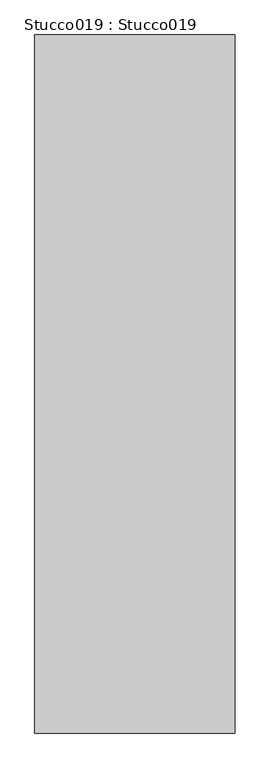
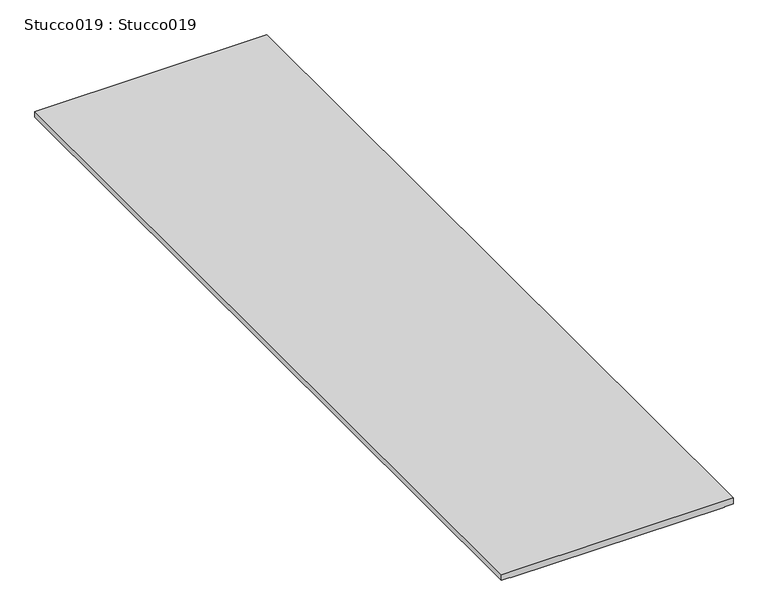
"""IFC4 building model written with IfcOpenShell, lengths in millimetres: proxy geometry, Stucco019 : Stucco019."""

import ifcopenshell
import ifcopenshell.guid

model = None  # the IFC model being written
_history = None  # IfcOwnerHistory: only IFC2X3 demands one
_inside = {}  # id of a spatial element -> (the spatial element, [elements in it])
_under = {}  # id of a project, library or spatial element -> (it, [spatial elements below it])
_declared = {}  # id of a project -> (the project, [libraries it declares])
_typed = {}  # id of a type object -> (the type object, [elements of that type])
_made_of = {}  # id of a material, layer set ... -> (it, [elements and type objects made of it])


def new_model(schema):
    """Start an empty IFC model of exactly this schema.

    Asked for "IFC4X3", IfcOpenShell would pick the latest addendum, in which some entities
    have other attributes; the version numbers below select the first issue.
    IFC2X3 requires an IfcOwnerHistory on every rooted entity: one is made here for all.
    """
    global model, _history
    if schema == "IFC4X3":
        model = ifcopenshell.file(schema_version=(4, 3, 0, 0))
    else:
        model = ifcopenshell.file(schema=schema)
    _inside.clear()
    _under.clear()
    _declared.clear()
    _typed.clear()
    _made_of.clear()
    _history = None
    if model.schema == "IFC2X3":
        org = make("IfcOrganization", Name="unknown")
        user = make(
            "IfcPersonAndOrganization",
            ThePerson=make("IfcPerson", FamilyName="unknown"),
            TheOrganization=org,
        )
        app = make(
            "IfcApplication",
            ApplicationDeveloper=org,
            Version="unknown",
            ApplicationFullName="unknown",
            ApplicationIdentifier="unknown",
        )
        _history = make(
            "IfcOwnerHistory",
            OwningUser=user,
            OwningApplication=app,
            ChangeAction="ADDED",
            CreationDate=0,
        )
    return model


def make(cls, **values):
    """One entity of the class cls with the attributes given. An attribute that is None is left unset."""
    return model.create_entity(
        cls, **{name: value for name, value in values.items() if value is not None}
    )


def rooted(cls, **values):
    """An entity with a GlobalId (a new one), such as an element, a storey or a relation."""
    return make(cls, GlobalId=ifcopenshell.guid.new(), OwnerHistory=_history, **values)


def si_unit(unit_type, name, prefix=None):
    """IfcSIUnit, for example si_unit("LENGTHUNIT", "METRE", prefix="MILLI")."""
    return make("IfcSIUnit", UnitType=unit_type, Prefix=prefix, Name=name)


def assignment(units):
    """IfcUnitAssignment: the units of a project."""
    return None if units is None else make("IfcUnitAssignment", Units=units)


def point(xyz):
    """IfcCartesianPoint."""
    return None if xyz is None else make("IfcCartesianPoint", Coordinates=xyz)


def direction(xyz):
    """IfcDirection."""
    return None if xyz is None else make("IfcDirection", DirectionRatios=xyz)


def frame(location, z_axis=None, x_axis=None):
    """IfcAxis2Placement3D, a coordinate frame: its origin and axes. An axis left out is left unset."""
    return make(
        "IfcAxis2Placement3D",
        Location=point(location),
        Axis=direction(z_axis),
        RefDirection=direction(x_axis),
    )


def origin():
    """The frame at (0, 0, 0) with its axes left unset."""
    return frame((0.0, 0.0, 0.0))


def place(relative_to, where):
    """IfcLocalPlacement: puts the frame where relative to a parent placement (None: the world)."""
    return make(
        "IfcLocalPlacement", PlacementRelTo=relative_to, RelativePlacement=where
    )


def context(
    kind, dimensions, precision=None, world=None, true_north=None, identifier=None
):
    """IfcGeometricRepresentationContext, for example the 3D "Model" context."""
    return make(
        "IfcGeometricRepresentationContext",
        ContextIdentifier=identifier,
        ContextType=kind,
        CoordinateSpaceDimension=dimensions,
        Precision=precision,
        WorldCoordinateSystem=world,
        TrueNorth=true_north,
    )


def project(units=None, contexts=None):
    """IfcProject with its units and contexts."""
    return rooted(
        "IfcProject",
        Name="project",
        RepresentationContexts=contexts,
        UnitsInContext=assignment(units),
    )


def spatial(cls, under=None, at=None, **own):
    """A site, building, storey or space (cls), placed at a placement, below another one or the project."""
    s = rooted(cls, ObjectPlacement=at, **own)
    if under is not None:
        _under.setdefault(under.id(), (under, []))[1].append(s)
    return s


def polyline(points):
    """IfcPolyline through the points."""
    return make("IfcPolyline", Points=[point(p) for p in points])


def outline(outer, holes=None, kind="AREA"):
    """IfcArbitraryClosedProfileDef: a profile drawn as a closed curve; with holes, ...WithVoids."""
    if holes is None:
        return make("IfcArbitraryClosedProfileDef", ProfileType=kind, OuterCurve=outer)
    return make(
        "IfcArbitraryProfileDefWithVoids",
        ProfileType=kind,
        OuterCurve=outer,
        InnerCurves=holes,
    )


def extrude(swept, where, along, depth):
    """IfcExtrudedAreaSolid: the profile swept, set in the frame where, extruded along a direction by depth."""
    return make(
        "IfcExtrudedAreaSolid",
        SweptArea=swept,
        Position=where,
        ExtrudedDirection=direction(along),
        Depth=depth,
    )


def shape(context_of_items, identifier, shape_type, items):
    """IfcShapeRepresentation: the items that make up one representation, for example the "Body"."""
    return make(
        "IfcShapeRepresentation",
        ContextOfItems=context_of_items,
        RepresentationIdentifier=identifier,
        RepresentationType=shape_type,
        Items=items,
    )


def source(mapping_origin, context_of_items, identifier, shape_type, items):
    """IfcRepresentationMap: a shape defined once, which mapped items show again and again."""
    return make(
        "IfcRepresentationMap",
        MappingOrigin=mapping_origin,
        MappedRepresentation=shape(context_of_items, identifier, shape_type, items),
    )


def transform(
    local_origin,
    x_axis=None,
    y_axis=None,
    z_axis=None,
    scale=None,
    scale2=None,
    scale3=None,
    uniform=True,
):
    """IfcCartesianTransformationOperator3D, or its non-uniform kind. x_axis, y_axis, z_axis: its Axis1, 2, 3."""
    if uniform:
        return make(
            "IfcCartesianTransformationOperator3D",
            Axis1=direction(x_axis),
            Axis2=direction(y_axis),
            LocalOrigin=point(local_origin),
            Scale=scale,
            Axis3=direction(z_axis),
        )
    return make(
        "IfcCartesianTransformationOperator3DnonUniform",
        Axis1=direction(x_axis),
        Axis2=direction(y_axis),
        LocalOrigin=point(local_origin),
        Scale=scale,
        Axis3=direction(z_axis),
        Scale2=scale2,
        Scale3=scale3,
    )


def mapped(mapping_source, mapping_target):
    """IfcMappedItem: shows the shape of a source again, moved by a transform."""
    return make(
        "IfcMappedItem", MappingSource=mapping_source, MappingTarget=mapping_target
    )


def made_of(thing, what):
    """Note that an element or type object is made of a material, layer set ...; save() writes the relation."""
    if what is not None:
        _made_of.setdefault(what.id(), (what, []))[1].append(thing)
    return thing


def element(
    cls,
    number,
    at=None,
    inside=None,
    cuts=None,
    type_object=None,
    material=None,
    context=None,
    identifier="Body",
    shape_type=None,
    held_by="IfcProductDefinitionShape",
    body=None,
    shapes=None,
    **own,
):
    """One element of the class cls, such as IfcWall. Its Tag is "e" and its number.

    at: its placement. inside: the storey or other place that contains it. cuts: it is an
    opening in that element (IfcRelVoidsElement). A single representation is given by context,
    identifier, shape_type and body (its items); several are given by shapes. held_by: the class
    of the entity that holds the representations. save() writes the other relations.
    """
    e = rooted(cls, Tag="e%d" % number, ObjectPlacement=at, **own)
    if body is not None:
        shapes = [shape(context, identifier, shape_type, body)]
    if shapes is not None:
        e.Representation = make(held_by, Representations=shapes)
    if inside is not None:
        _inside.setdefault(inside.id(), (inside, []))[1].append(e)
    if cuts is not None:
        rooted(
            "IfcRelVoidsElement", RelatingBuildingElement=cuts, RelatedOpeningElement=e
        )
    if type_object is not None:
        _typed.setdefault(type_object.id(), (type_object, []))[1].append(e)
    return made_of(e, material)


def aggregate(whole, parts):
    """IfcRelAggregates: a whole, such as a stair, and the parts it consists of."""
    return rooted("IfcRelAggregates", RelatingObject=whole, RelatedObjects=parts)


def save(model, path):
    """Write the relations noted so far, then the file.

    IfcRelAggregates (storeys below a building ...), IfcRelContainedInSpatialStructure (elements
    in a storey), IfcRelDefinesByType, IfcRelAssociatesMaterial and IfcRelDeclares: one each for
    every whole, place, type object, material and project.
    """
    for whole, parts in _under.values():
        aggregate(whole, parts)
    for where, things in _inside.values():
        rooted(
            "IfcRelContainedInSpatialStructure",
            RelatedElements=things,
            RelatingStructure=where,
        )
    for kind, things in _typed.values():
        rooted("IfcRelDefinesByType", RelatedObjects=things, RelatingType=kind)
    for what, things in _made_of.values():
        rooted("IfcRelAssociatesMaterial", RelatedObjects=things, RelatingMaterial=what)
    for by, libraries in _declared.values():
        rooted("IfcRelDeclares", RelatingContext=by, RelatedDefinitions=libraries)
    model.write(path)


def stucco019_stucco019_f4d67199(model_context):
    return source(origin(), model_context, "Body", "SweptSolid", [
        extrude(outline(polyline([(39545.1675708, -7190.9913235), (39543.8875708, -7190.9913235), (39543.8875708, -6662.3408502), (39545.1675708, -6662.3408502), (39545.1675708, -6639.9076663), (39560.2460083, -6639.9076663), (39560.2460083, -7213.4245075), (39545.1675708, -7213.4245075), (39545.1675708, -7190.9913235)])), frame((0.0, 7982.1531721, 0.0), z_axis=(0.0, 1.0, 0.0), x_axis=(0.0, 0.0, 1.0)), (0.0, 0.0, 1.0), 2000.0),
    ])


if __name__ == "__main__":
    model = new_model("IFC4")
    model_context = context("Model", 3, world=origin())
    ifc_project = project(units=[si_unit("LENGTHUNIT", "METRE", prefix="MILLI")], contexts=[model_context])
    site = spatial("IfcSite", under=ifc_project)
    building = spatial("IfcBuilding", under=site)
    placement = place(None, origin())
    stucco019_stucco019_shape = stucco019_stucco019_f4d67199(model_context)
    element("IfcBuildingElementProxy", 1, Name="Stucco019 : Stucco019", ObjectType="Stucco019 : Stucco019", at=placement, inside=building, context=model_context, shape_type="MappedRepresentation", body=[
        mapped(stucco019_stucco019_shape, transform((0.0, 0.0, 0.0), x_axis=(1.0, 0.0, 0.0), y_axis=(0.0, 1.0, 0.0), z_axis=(0.0, 0.0, 1.0))),
    ])
    save(model, "model.ifc")

# Revit data of these elements
# Type "Stucco019 : Stucco019"
#   NameOverride = "Stucco019"
# Element 1 (IfcBuildingElementProxy, "Stucco019 : Stucco019")
#   Materials on its faces: "7/8\" SMOOTH TROWEL EXTERIOR STUCCO"
# Materials
#   "7/8\" SMOOTH TROWEL EXTERIOR STUCCO": class "Unassigned", colour RGB 255 255 255, transparency 0, Cost = 0
